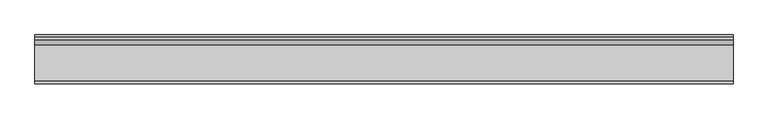
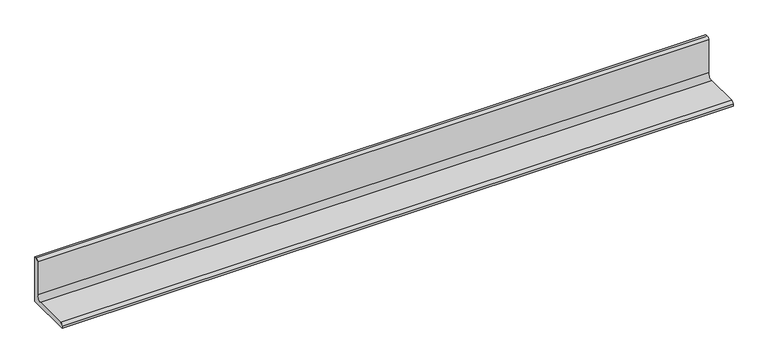
"""IFC4 building model written with IfcOpenShell, lengths in millimetres: beam geometry, NLRS_28_SF_LIB_stalen ligger hoekprofiel gelijkzijdig-AV-MMBS-SRP_gen_rsf : stalen ligger gelijkzijdig hoekprofiel LEQU_gen__150x150x15."""

from ifc_helpers import new_model, si_unit, point, frame, frame_2d, origin, place, context, project, spatial, polyline, circle_curve, trimmed, segment, composite_curve, outline, extrude, source, transform, mapped, element, save


def beam_d577a1de(model_context):
    return source(origin(), model_context, "Body", "SweptSolid", [
        extrude(outline(composite_curve([segment(polyline([(42.5, -42.5), (-107.5, -42.5), (-107.5, -35.5)]), True, "CONTINUOUS"), segment(trimmed(circle_curve(frame_2d((-99.5, -35.5)), 8.0), [point((-107.5, -35.5))], [point((-99.5, -27.5))], False, "CARTESIAN"), True, "CONTINUOUS"), segment(polyline([(-99.5, -27.5), (11.5, -27.5)]), True, "CONTINUOUS"), segment(trimmed(circle_curve(frame_2d((11.5, -11.5)), 16.0), [point((11.5, -27.5))], [point((27.5, -11.5))], True, "CARTESIAN"), True, "CONTINUOUS"), segment(polyline([(27.5, -11.5), (27.5, 99.5)]), True, "CONTINUOUS"), segment(trimmed(circle_curve(frame_2d((35.5, 99.5)), 8.0), [point((27.5, 99.5))], [point((35.5, 107.5))], False, "CARTESIAN"), True, "CONTINUOUS"), segment(polyline([(35.5, 107.5), (42.5, 107.5), (42.5, -42.5)]), True, "CONTINUOUS")], self_intersect=False)), frame((-1070.0, 0.0, 0.0), z_axis=(1.0, 0.0, 0.0), x_axis=(0.0, 1.0, 0.0)), (0.0, 0.0, 1.0), 2140.0),
    ])


if __name__ == "__main__":
    model = new_model("IFC4")
    model_context = context("Model", 3, world=origin())
    ifc_project = project(units=[si_unit("LENGTHUNIT", "METRE", prefix="MILLI")], contexts=[model_context])
    site = spatial("IfcSite", under=ifc_project)
    building = spatial("IfcBuilding", under=site)
    placement = place(None, origin())
    beam_shape = beam_d577a1de(model_context)
    element("IfcBeam", 1, ObjectType="NLRS_28_SF_LIB_stalen ligger hoekprofiel gelijkzijdig-AV-MMBS-SRP_gen_rsf : stalen ligger gelijkzijdig hoekprofiel LEQU_gen__150x150x15", at=placement, inside=building, context=model_context, shape_type="MappedRepresentation", body=[
        mapped(beam_shape, transform((0.0, 0.0, 0.0), x_axis=(1.0, 0.0, 0.0), y_axis=(0.0, 1.0, 0.0), z_axis=(0.0, 0.0, 1.0))),
    ])
    save(model, "model.ifc")

# Revit data of these elements
# Type "NLRS_28_SF_LIB_stalen ligger hoekprofiel gelijkzijdig-AV-MMBS-SRP_gen_rsf : stalen ligger gelijkzijdig hoekprofiel LEQU_gen__150x150x15"
#   Type IfcGUID = "2CEqVLPNH8KRN7ghwV3a1U"
#   IfcExportAs = "IfcBeamType"
#   Type Comments = "L150x150x15"
#   Model = " "
#   Manufacturer = " "
#   Fire Rating = " "
#   Description = "stalen ligger L150x150x15"
#   Assembly Code = "28.11"
#   vz = 107.5 mm
#   vy = 107.5 mm
#   tw = 15 mm
#   tf = 15 mm
#   ri = 8 mm
#   ra = 16 mm
#   d = 150 mm
#   bf = 150 mm
#   NLRS_C_lengte [instance default] = 1524 mm
#   Length [instance default] = 1524 mm
#   Structural Material = NLRS_h2_staal_gen_rsf
#   Keynote = ""
# Element 1 (IfcBeam, "NLRS_28_SF_LIB_stalen ligger hoekprofiel gelijkzijdig-AV-MMBS-SRP_gen_rsf : stalen ligger gelijkzijdig hoekprofiel LEQU_gen__150x150x15")
#   NLRS_C_lengte = 2140 mm
#   Materials on its faces: "NLRS_h2_staal_gen_rsf"
# Materials
#   "NLRS_h2_staal_gen_rsf": class "H - Metaal", colour RGB 189 187 185, transparency 0, Keynote = "h2", Manufacturer = "Revit Standards Foundation", URL = "www.revitstandards.org", Description = "staal", Cost = 0
